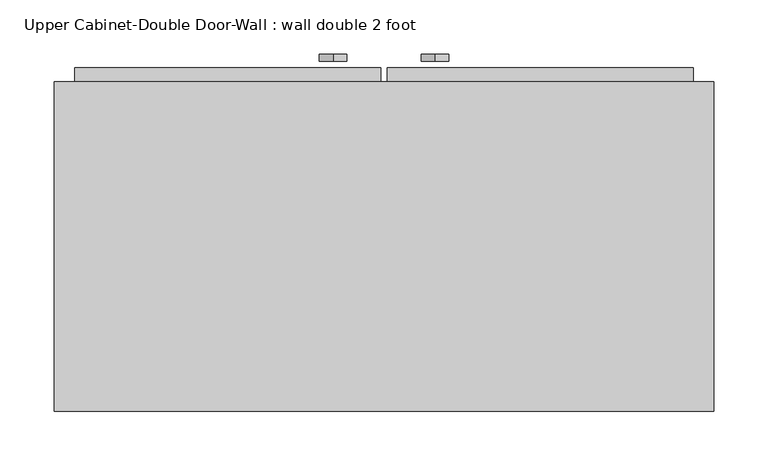
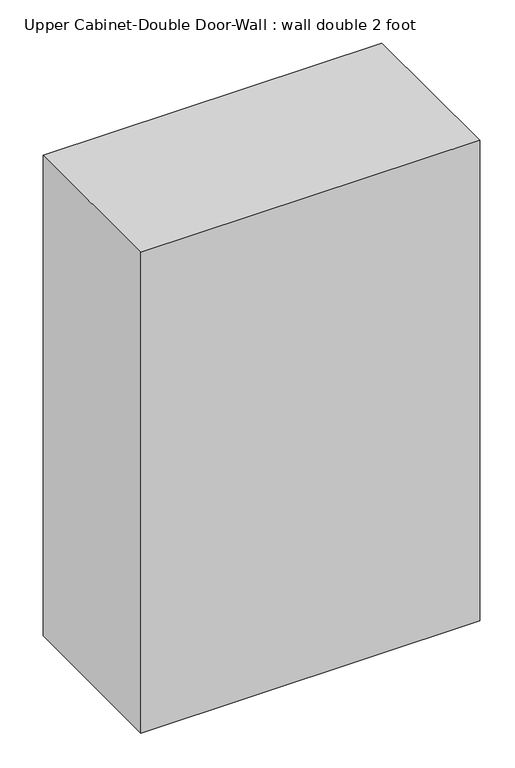
"""IFC4 building model written with IfcOpenShell, lengths in millimetres: furniture geometry, Upper Cabinet-Double Door-Wall : wall double 2 foot."""

from ifc_helpers import new_model, si_unit, point, frame, frame_2d, origin, place, context, project, spatial, polyline, circle_curve, trimmed, segment, composite_curve, outline, extrude, faceted_brep, source, transform, mapped, element, save


def upper_cabinet_double_door_wall_wall_double_2_foot_255d7463(model_context):
    return source(origin(), model_context, "Body", "SolidModel", [
        faceted_brep([(-275.0288372, 56.35625, 2133.6), (-275.0288372, 56.35625, 1219.2), (334.5711628, 56.35625, 1219.2), (334.5711628, 56.35625, 2133.6), (-275.0288372, 361.15625, 2133.6), (334.5711628, 361.15625, 2133.6), (334.5711628, 361.15625, 1219.2), (-275.0288372, 361.15625, 1219.2), (-255.9788372, 361.15625, 2114.55), (-255.9788372, 361.15625, 1238.25), (315.5211628, 361.15625, 1238.25), (315.5211628, 361.15625, 2114.55), (315.5211628, 75.40625, 2114.55), (-255.9788372, 75.40625, 2114.55), (315.5211628, 75.40625, 1238.25), (-255.9788372, 75.40625, 1238.25)], [[[0, 1, 2, 3]], [[4, 5, 6, 7], [8, 9, 10, 11]], [[1, 0, 4, 7]], [[2, 1, 7, 6]], [[3, 2, 6, 5]], [[0, 3, 5, 4]], [[8, 11, 12, 13]], [[11, 10, 14, 12]], [[10, 9, 15, 14]], [[9, 8, 13, 15]], [[13, 12, 14, 15]]]),
        extrude(outline(polyline([(32.9461628, 373.85625), (315.5211628, 373.85625), (315.5211628, 342.10625), (32.9461628, 342.10625), (32.9461628, 373.85625)])), frame((0.0, 0.0, 1238.25), z_axis=(0.0, 0.0, 1.0), x_axis=(1.0, 0.0, 0.0)), (0.0, 0.0, 1.0), 876.3),
        extrude(outline(polyline([(-255.9788372, 373.85625), (26.5961628, 373.85625), (26.5961628, 342.10625), (-255.9788372, 342.10625), (-255.9788372, 373.85625)])), frame((0.0, 0.0, 1238.25), z_axis=(0.0, 0.0, 1.0), x_axis=(1.0, 0.0, 0.0)), (0.0, 0.0, 1.0), 876.3),
        extrude(outline(composite_curve([segment(trimmed(circle_curve(frame_2d((1381.4214732, 76.8007051)), 12.7), [point((1368.7214732, 76.8007051))], [point((1394.1214732, 76.8007051))], False, "CARTESIAN"), True, "CONTINUOUS"), segment(trimmed(circle_curve(frame_2d((1381.4214732, 76.8007051)), 12.7), [point((1394.1214732, 76.8007051))], [point((1368.7214732, 76.8007051))], False, "CARTESIAN"), True, "CONTINUOUS")], self_intersect=False)), frame((0.0, 380.20625, 0.0), z_axis=(0.0, 1.0, 0.0), x_axis=(0.0, 0.0, 1.0)), (0.0, 0.0, 1.0), 6.35),
        extrude(outline(composite_curve([segment(trimmed(circle_curve(frame_2d((1381.4214732, -17.2583796)), 12.7), [point((1368.7214732, -17.2583796))], [point((1394.1214732, -17.2583796))], False, "CARTESIAN"), True, "CONTINUOUS"), segment(trimmed(circle_curve(frame_2d((1381.4214732, -17.2583796)), 12.7), [point((1394.1214732, -17.2583796))], [point((1368.7214732, -17.2583796))], False, "CARTESIAN"), True, "CONTINUOUS")], self_intersect=False)), frame((0.0, 380.20625, 0.0), z_axis=(0.0, 1.0, 0.0), x_axis=(0.0, 0.0, 1.0)), (0.0, 0.0, 1.0), 6.35),
    ])


if __name__ == "__main__":
    model = new_model("IFC4")
    model_context = context("Model", 3, world=origin())
    ifc_project = project(units=[si_unit("LENGTHUNIT", "METRE", prefix="MILLI")], contexts=[model_context])
    site = spatial("IfcSite", under=ifc_project)
    building = spatial("IfcBuilding", under=site)
    placement = place(None, origin())
    upper_cabinet_double_door_wall_wall_double_2_foot_shape = upper_cabinet_double_door_wall_wall_double_2_foot_255d7463(model_context)
    element("IfcFurniture", 1, ObjectType="Upper Cabinet-Double Door-Wall : wall double 2 foot", at=placement, inside=building, context=model_context, shape_type="MappedRepresentation", body=[
        mapped(upper_cabinet_double_door_wall_wall_double_2_foot_shape, transform((0.0, 0.0, 0.0), x_axis=(1.0, 0.0, 0.0), y_axis=(0.0, 1.0, 0.0), z_axis=(0.0, 0.0, 1.0))),
    ])
    save(model, "model.ifc")

# Revit data of these elements
# Type "Upper Cabinet-Double Door-Wall : wall double 2 foot"
#   Assembly Code = "C1030410"
#   Depth = 1' - 0"
#   Height = 3' - 0"
#   Top Of Cabinet = 7' - 0"
#   Width = 2' - 0"
#   Cabinet Material = Base cabinet 2120100 Aspekt - 83012120100 - White
#   Door/Drawer Material = Base cabinet 2120100 Aspekt - 83012120100 - White
#   Handle Material = Cabinets - Handles
#   Default Elevation = 0
# Element 1 (IfcFurniture, "Upper Cabinet-Double Door-Wall : wall double 2 foot")
#   Materials on its faces: "Base cabinet 2120100 Aspekt - 83012120100 - White"
# Materials
#   "Base cabinet 2120100 Aspekt - 83012120100 - White": class "Miscellaneous", colour RGB 255 255 255, transparency 0, Manufacturer = "Marbodal", URL = "http://www.marbodal.se", Cost = 0
#   "Cabinets - Handles": class "Metal", colour RGB 57 57 57, transparency 0
